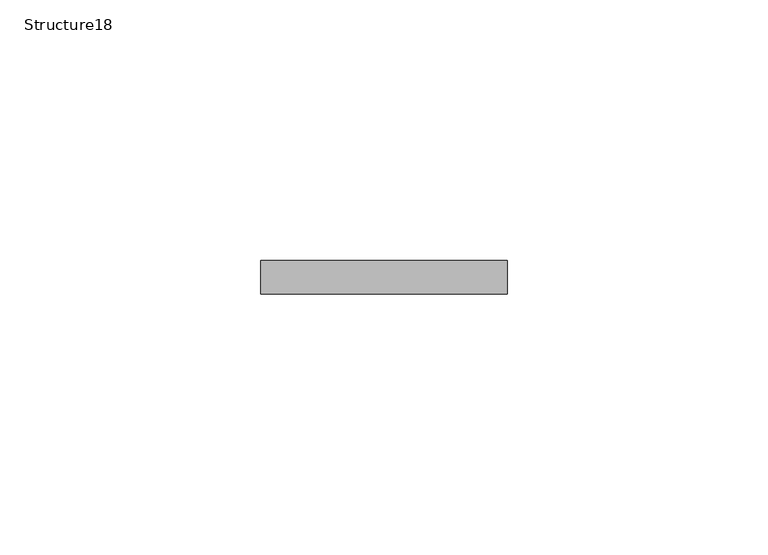
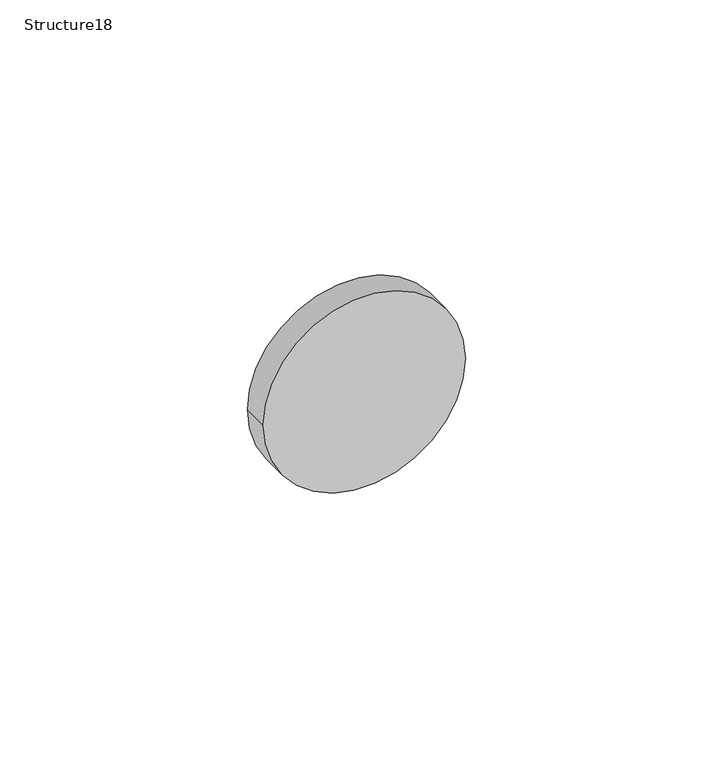
"""IFC4 building model written with IfcOpenShell, lengths in millimetres: proxy geometry, Structure18 : Structure668217139."""

from ifc_helpers import new_model, si_unit, point, frame, frame_2d, origin, place, context, project, spatial, circle_curve, trimmed, segment, composite_curve, outline, extrude, source, transform, mapped, element, save


def structure18_2cee4dc9(model_context):
    return source(origin(), model_context, "Body", "SweptSolid", [
        extrude(outline(composite_curve([segment(trimmed(circle_curve(frame_2d((39371.6422813, 7343.0332877)), 23.5716554), [point((39371.6422813, 7319.4616323))], [point((39371.6422813, 7366.6049431))], False, "CARTESIAN"), True, "CONTINUOUS"), segment(trimmed(circle_curve(frame_2d((39371.6422813, 7343.0332877)), 23.5716554), [point((39371.6422813, 7366.6049431))], [point((39371.6422813, 7319.4616323))], False, "CARTESIAN"), True, "CONTINUOUS")], self_intersect=False)), frame((0.0, 1928.1961961, 0.0), z_axis=(0.0, 1.0, 0.0), x_axis=(0.0, 0.0, 1.0)), (0.0, 0.0, 1.0), 6.35),
    ])


if __name__ == "__main__":
    model = new_model("IFC4")
    model_context = context("Model", 3, world=origin())
    ifc_project = project(units=[si_unit("LENGTHUNIT", "METRE", prefix="MILLI")], contexts=[model_context])
    site = spatial("IfcSite", under=ifc_project)
    building = spatial("IfcBuilding", under=site)
    placement = place(None, origin())
    structure18_shape = structure18_2cee4dc9(model_context)
    element("IfcBuildingElementProxy", 1, Name="Structure18 : Structure668217139", ObjectType="Structure18 : Structure668217139", at=placement, inside=building, context=model_context, shape_type="MappedRepresentation", body=[
        mapped(structure18_shape, transform((0.0, 0.0, 0.0), x_axis=(1.0, 0.0, 0.0), y_axis=(0.0, 1.0, 0.0), z_axis=(0.0, 0.0, 1.0))),
    ])
    save(model, "model.ifc")

# Revit data of these elements
# Type "Structure18 : Structure668217139"
#   NameOverride = "Structure668217139"
# Element 1 (IfcBuildingElementProxy, "Structure18 : Structure668217139")
#   Materials on its faces: "RUBBER GASKET"
# Materials
#   "RUBBER GASKET": class "Unassigned", colour RGB 70 70 70, transparency 0
